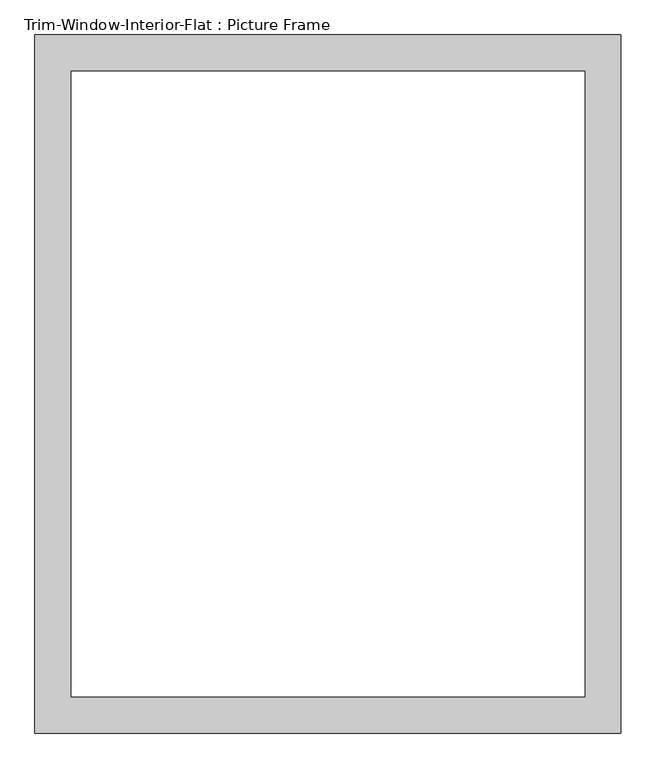
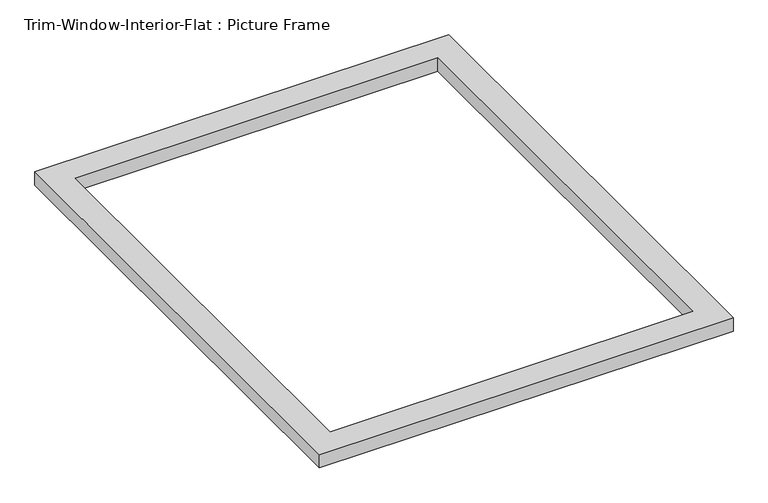
"""IFC4 building model written with IfcOpenShell, lengths in millimetres: proxy geometry, Trim-Window-Interior-Flat : Picture Frame."""

from ifc_helpers import new_model, si_unit, origin, origin_with_axes, place, context, project, spatial, polyline, outline, extrude, source, transform, mapped, element, save


def trim_window_interior_flat_picture_frame_6b7ff15f(model_context):
    return source(origin(), model_context, "Body", "SweptSolid", [
        extrude(outline(polyline([(463.55, -44.45), (-463.55, -44.45), (-463.55, 1060.45), (463.55, 1060.45), (463.55, -44.45)]), holes=[polyline([(406.4, 12.7), (406.4, 1003.3), (-406.4, 1003.3), (-406.4, 12.7), (406.4, 12.7)])]), origin_with_axes(), (0.0, 0.0, 1.0), 31.75),
    ])


if __name__ == "__main__":
    model = new_model("IFC4")
    model_context = context("Model", 3, world=origin())
    ifc_project = project(units=[si_unit("LENGTHUNIT", "METRE", prefix="MILLI")], contexts=[model_context])
    site = spatial("IfcSite", under=ifc_project)
    building = spatial("IfcBuilding", under=site)
    placement = place(None, origin())
    trim_window_interior_flat_picture_frame_shape = trim_window_interior_flat_picture_frame_6b7ff15f(model_context)
    element("IfcBuildingElementProxy", 1, Name="Trim-Window-Interior-Flat : Picture Frame", ObjectType="Trim-Window-Interior-Flat : Picture Frame", at=placement, inside=building, context=model_context, shape_type="MappedRepresentation", body=[
        mapped(trim_window_interior_flat_picture_frame_shape, transform((0.0, 0.0, 0.0), x_axis=(1.0, 0.0, 0.0), y_axis=(0.0, 1.0, 0.0), z_axis=(0.0, 0.0, 1.0))),
    ])
    save(model, "model.ifc")

# Revit data of these elements
# Type "Trim-Window-Interior-Flat : Picture Frame"
#   Trim Thickness_Picture Frame = 0' - 1 1/4"
#   Trim Width = 0' - 2 1/4"
#   Trim Thickness_with Sill = 0' - 0 3/4"
#   Sill Thickness = 0' - 1 1/4"
#   Opening Width [instance default] = 2' - 0"
#   Opening Height [instance default] = 3' - 0"
#   Default Elevation = 4' - 0"
#   Sill = no
#   Picture Frame = yes
#   Trim Material [instance default] = none
# Element 1 (IfcBuildingElementProxy, "Trim-Window-Interior-Flat : Picture Frame")
#   Opening Width = 2' - 9"
#   Opening Height = 3' - 4"
#   Trim Material = Wood - Stained
#   Materials on its faces: "Wood - Stained"
# Materials
#   "Wood - Stained": class "Wood", colour RGB 224 178 126, transparency 0, Cost = 0
